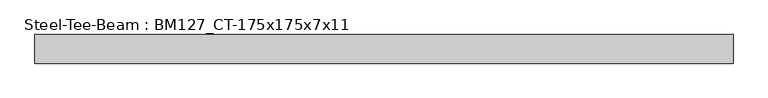
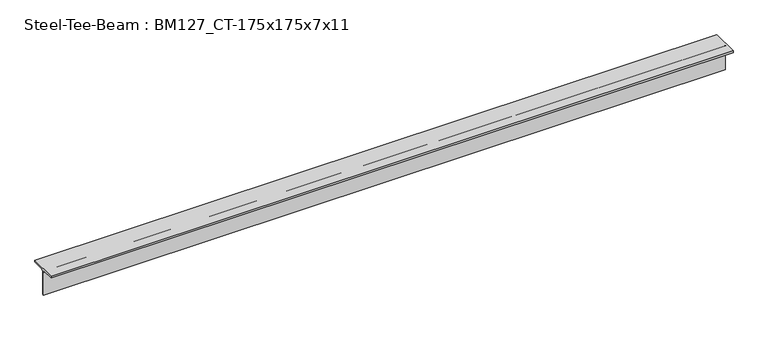
"""IFC4 building model written with IfcOpenShell, lengths in millimetres: beam geometry, Steel-Tee-Beam : BM127_CT-175x175x7x11."""

from ifc_helpers import new_model, si_unit, point, frame, frame_2d, origin, place, context, project, spatial, polyline, circle_curve, trimmed, segment, composite_curve, outline, extrude, source, transform, mapped, element, save


def steel_tee_beam_bm127_ct_175x175x7x11_f7a1ba5a(model_context):
    return source(origin(), model_context, "Body", "SweptSolid", [
        extrude(outline(composite_curve([segment(polyline([(-87.5, 87.5), (87.5, 87.5), (87.5, 76.5), (17.5, 76.5)]), True, "CONTINUOUS"), segment(trimmed(circle_curve(frame_2d((17.5, 62.5)), 14.0), [point((17.5, 76.5))], [point((3.5, 62.5))], True, "CARTESIAN"), True, "CONTINUOUS"), segment(polyline([(3.5, 62.5), (3.5, -87.5), (-3.5, -87.5), (-3.5, 62.5)]), True, "CONTINUOUS"), segment(trimmed(circle_curve(frame_2d((-17.5, 62.5)), 14.0), [point((-3.5, 62.5))], [point((-17.5, 76.5))], True, "CARTESIAN"), True, "CONTINUOUS"), segment(polyline([(-17.5, 76.5), (-87.5, 76.5), (-87.5, 87.5)]), True, "CONTINUOUS")], self_intersect=False)), frame((-2078.5248279, 0.0, 0.0), z_axis=(1.0, 0.0, 0.0), x_axis=(0.0, 1.0, 0.0)), (0.0, 0.0, 1.0), 4262.7315887),
    ])


if __name__ == "__main__":
    model = new_model("IFC4")
    model_context = context("Model", 3, world=origin())
    ifc_project = project(units=[si_unit("LENGTHUNIT", "METRE", prefix="MILLI")], contexts=[model_context])
    site = spatial("IfcSite", under=ifc_project)
    building = spatial("IfcBuilding", under=site)
    placement = place(None, origin())
    steel_tee_beam_bm127_ct_175x175x7x11_shape = steel_tee_beam_bm127_ct_175x175x7x11_f7a1ba5a(model_context)
    element("IfcBeam", 1, ObjectType="Steel-Tee-Beam : BM127_CT-175x175x7x11", at=placement, inside=building, context=model_context, shape_type="MappedRepresentation", body=[
        mapped(steel_tee_beam_bm127_ct_175x175x7x11_shape, transform((0.0, 0.0, 0.0), x_axis=(1.0, 0.0, 0.0), y_axis=(0.0, 1.0, 0.0), z_axis=(0.0, 0.0, 1.0))),
    ])
    save(model, "model.ifc")

# Revit data of these elements
# Type "Steel-Tee-Beam : BM127_CT-175x175x7x11"
#   Surface Area = 0.00 m²/m
#   Section Area = 31.57 cm²
#   Mass per Unit Length = 24.80 kg/m
#   Length [instance default] = 1524 mm
#   bf = 175 mm
#   d = 175 mm
#   k = 25 mm
#   kr = 14 mm
#   tf = 11 mm
#   tw = 7 mm
#   hec_material4 [instance default] = none
#   hec_material3 [instance default] = none
#   hec_material2 [instance default] = none
#   hec_material1 [instance default] = none
#   Structural Material [instance default] = Steel, 45-345
#   Assembly Code = ""
# Element 1 (IfcBeam, "Steel-Tee-Beam : BM127_CT-175x175x7x11")
#   hec_material3 = F01AC000-00002_Building/Shelter Fire Proofing Work_Intumescent Coating Type_1 hr. rating (UL 1709))
#   hec_material2 = S01AA010-00002_Main Steel Structure Fabrication Work_Shelter/Building_Steel Painting/Coating_for Fireproofed Steel Surface, Surface Preparation & Primer Coat
#   hec_material1 = S03AA029-00001_Main Steel Structure Erection Work_Shelter/Building_Light Steel
#   Structural Material = S01AA003-00001_Main Steel Structure Fabrication Work_Shelter/Building_Light Steel - Standard
#   Materials on its faces: "S01AA003-00001_Main Steel Structure Fabrication Work_Shelter/Building_Light Steel - Standard"
# Materials
#   "Steel, 45-345": class "Metal", colour RGB 189 187 185, transparency 0, Description = "Steel 345 MPa", Cost = 0
#   "S01AA003-00001_Main Steel Structure Fabrication Work_Shelter/Building_Light Steel - Standard": class "Metal", colour RGB 120 120 120, transparency 0, Comments = "(30KG/M>Weight)", Description = "Structural steel 50ksi", W00) Work Master Code = "S01AA003-00001", W01) Work Master_Lv1 = "Main Steel Structure Fabrication Work", W02) Work Master_Lv2 = "Shelter/Building", W03) Work Master_Spec.1 = "Light Steel - Standard (30KG/M>Weight)", Cost = 0
#   "F01AC000-00002_Building/Shelter Fire Proofing Work_Intumescent Coating Type_1 hr. rating (UL 1709))": class "Metal", colour RGB 255 128 128, transparency 0, Description = "Paint finished steel", W00) Work Master Code = "F01AC000-00002", W01) Work Master_Lv1 = "Building/Shelter Fire Proofing Work", W02) Work Master_Lv2 = "Intumescent Coating Type", W03) Work Master_Spec.1 = "1 hr. rating (UL 1709)", Cost = 0
#   "S01AA010-00002_Main Steel Structure Fabrication Work_Shelter/Building_Steel Painting/Coating_for Fireproofed Steel Surface, Surface Preparation & Primer Coat": class "Metal", colour RGB 120 120 120, transparency 0, Description = "Paint finished steel", W00) Work Master Code = "SS01AA010-00002", W01) Work Master_Lv1 = "Main Steel Structure Fabrication Work", W02) Work Master_Lv2 = "Shelter/Building", W03) Work Master_Spec.1 = "Steel Painting/Coating", W04) Work Master_Spec.2 = "for Fireproofed Steel Surface, Surface Preparation & Primer Coat", Cost = 0
#   "S03AA029-00001_Main Steel Structure Erection Work_Shelter/Building_Light Steel": class "Metal", colour RGB 120 120 120, transparency 0, Comments = "(30KG/M>Weight)", Description = "Structural steel 50ksi", W00) Work Master Code = "S03AA029-00001", W01) Work Master_Lv1 = "Main Steel Structure Erection Work", W02) Work Master_Lv2 = "Shelter/Building", W03) Work Master_Spec.1 = "Light Steel (30KG/M>Weight)", Cost = 0
